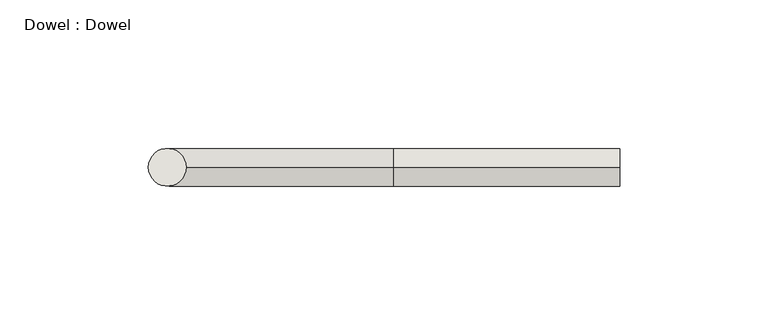
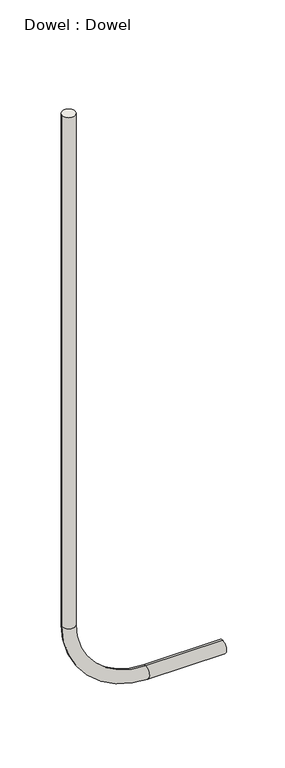
"""IFC4 building model written with IfcOpenShell, lengths in millimetres: wall geometry, Dowel : Dowel."""

from ifc_helpers import new_model, si_unit, point, frame, origin, place, context, project, spatial, circle_curve, ellipse_curve, trimmed, source, transform, mapped, element, save
from ifc_brep_helpers import plane_surface, cylinder_surface, revolved_surface, advanced_brep


def dowel_dowel_69415ce0(model_context):
    return source(origin(), model_context, "Body", "AdvancedBrep", [
        advanced_brep(
        [(430120.425, 825.5, 533.4), (430133.125, 825.5, 533.4), (430120.425, 825.5, 0.0), (430133.125, 825.5, 0.0), (430202.975, 825.5, -69.85), (430202.975, 825.5, -82.55), (430279.175, 825.5, -82.55), (430279.175, 825.5, -69.85)],
        [
            (0, 1, circle_curve(frame((430126.775, 825.5, 533.4), z_axis=(0.0, 0.0, 1.0), x_axis=(1.0, 0.0, 0.0)), 6.35)),
            (1, 0, circle_curve(frame((430126.775, 825.5, 533.4), z_axis=(0.0, 0.0, 1.0), x_axis=(1.0, 0.0, 0.0)), 6.35)),
            (0, 2),
            (2, 3, circle_curve(frame((430126.775, 825.5, 0.0), z_axis=(0.0, 0.0, 1.0), x_axis=(1.0, 0.0, 0.0)), 6.35)),
            (3, 1),
            (3, 2, circle_curve(frame((430126.775, 825.5, 0.0), z_axis=(0.0, 0.0, 1.0), x_axis=(1.0, 0.0, 0.0)), 6.35)),
            (4, 3, circle_curve(frame((430202.975, 825.5, 0.0), z_axis=(0.0, 1.0, 0.0), x_axis=(-1.0, 0.0, 0.0)), 69.85)),
            (2, 5, circle_curve(frame((430202.975, 825.5, 0.0), z_axis=(0.0, -1.0, 0.0), x_axis=(-1.0, 0.0, 0.0)), 82.55)),
            (5, 4, circle_curve(frame((430202.975, 825.5, -76.2), z_axis=(-1.0, 0.0, 0.0), x_axis=(0.0, 0.0, 1.0)), 6.35)),
            (4, 5, circle_curve(frame((430202.975, 825.5, -76.2), z_axis=(-1.0, 0.0, 0.0), x_axis=(0.0, 0.0, 1.0)), 6.35)),
            (6, 7, circle_curve(frame((430279.175, 825.5, -76.2), z_axis=(1.0, 0.0, 0.0), x_axis=(0.0, 0.0, 1.0)), 6.35)),
            (7, 6, circle_curve(frame((430279.175, 825.5, -76.2), z_axis=(1.0, 0.0, 0.0), x_axis=(0.0, 0.0, 1.0)), 6.35)),
            (5, 6),
            (7, 4),
        ],
        [
            plane_surface(frame((430126.775, 825.5, 533.4), z_axis=(0.0, 0.0, 1.0), x_axis=(0.0, -1.0, 0.0))),
            cylinder_surface(frame((430126.775, 825.5, 533.4), z_axis=(0.0, 0.0, 1.0), x_axis=(1.0, 0.0, 0.0)), 6.35),
            revolved_surface(trimmed(ellipse_curve(frame((430126.775, 825.5, 0.0), z_axis=(0.0, 0.0, 1.0), x_axis=(1.0, 0.0, 0.0)), 6.35, 6.35), [point((430120.425, 825.5, 0.0))], [point((430133.125, 825.5, 0.0))], True, "CARTESIAN"), (430202.975, 825.5, 0.0), (0.0, -1.0, 0.0)),
            revolved_surface(trimmed(ellipse_curve(frame((430126.775, 825.5, 0.0), z_axis=(0.0, 0.0, 1.0), x_axis=(1.0, 0.0, 0.0)), 6.35, 6.35), [point((430133.125, 825.5, 0.0))], [point((430120.425, 825.5, 0.0))], True, "CARTESIAN"), (430202.975, 825.5, 0.0), (0.0, -1.0, 0.0)),
            plane_surface(frame((430279.175, 825.5, -76.2), z_axis=(1.0, 0.0, 0.0), x_axis=(0.0, -1.0, 0.0))),
            cylinder_surface(frame((430202.975, 825.5, -76.2), z_axis=(-1.0, 0.0, 0.0), x_axis=(0.0, 0.0, 1.0)), 6.35),
        ],
        [
            (0, [[1, 2]]),
            (1, [[-1, 3, 4, 5]]),
            (1, [[-2, -5, 6, -3]]),
            (2, [[7, -4, 8, 9]]),
            (3, [[-8, -6, -7, 10]]),
            (4, [[11, 12]]),
            (5, [[-9, 13, -12, 14]]),
            (5, [[-10, -14, -11, -13]]),
        ],
    ),
    ])


if __name__ == "__main__":
    model = new_model("IFC4")
    model_context = context("Model", 3, world=origin())
    ifc_project = project(units=[si_unit("LENGTHUNIT", "METRE", prefix="MILLI")], contexts=[model_context])
    site = spatial("IfcSite", under=ifc_project)
    building = spatial("IfcBuilding", under=site)
    placement = place(None, origin())
    dowel_dowel_shape = dowel_dowel_69415ce0(model_context)
    element("IfcWall", 1, ObjectType="Dowel : Dowel", at=placement, inside=building, context=model_context, shape_type="MappedRepresentation", body=[
        mapped(dowel_dowel_shape, transform((0.0, 0.0, 0.0), x_axis=(1.0, 0.0, 0.0), y_axis=(0.0, 1.0, 0.0), z_axis=(0.0, 0.0, 1.0))),
    ])
    save(model, "model.ifc")

# Revit data of these elements
# Element 1 (IfcWall, "Dowel : Dowel")
#   Materials on its faces: "6\" CMU WALL W/#4 VERT. BARS AT 32\" O.C. (TYP.)"
# Materials
#   "6\" CMU WALL W/#4 VERT. BARS AT 32\" O.C. (TYP.)": class "Generic", colour RGB 255 255 255, transparency 0, Cost = 0
